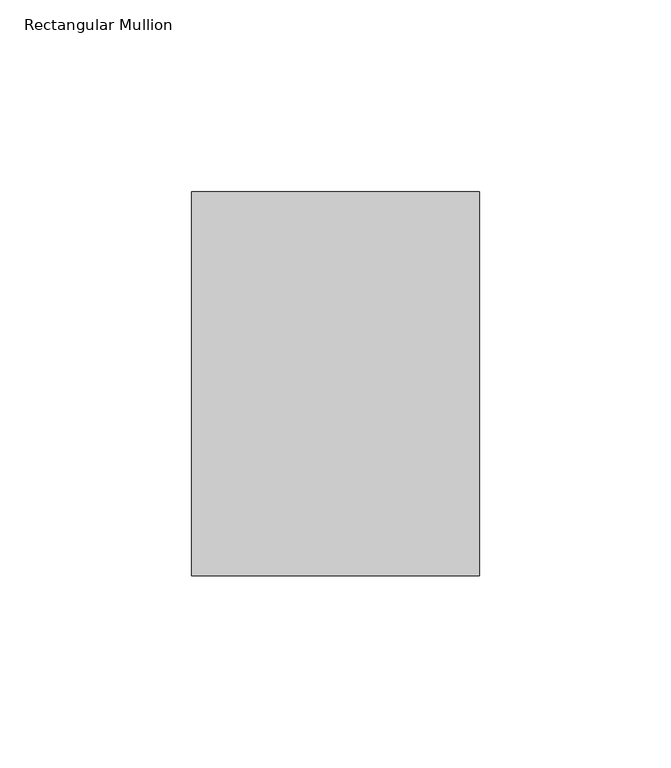
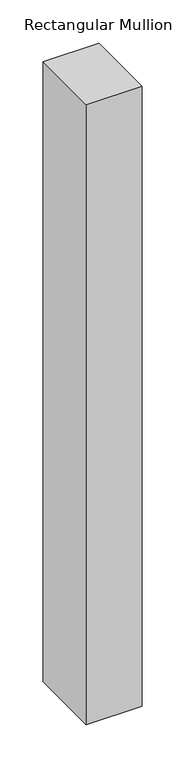
"""IFC4 building model written with IfcOpenShell, lengths in millimetres: member geometry, Rectangular Mullion : 알루미늄_Rectangular Cap_100 x 75."""

from ifc_helpers import new_model, si_unit, frame, origin, place, context, project, spatial, polyline, outline, extrude, source, transform, mapped, element, save


def rectangular_mullion_fe860069(model_context):
    return source(origin(), model_context, "Body", "SweptSolid", [
        extrude(outline(polyline([(0.0, 50.0), (0.0, -50.0), (-75.0, -50.0), (-75.0, 50.0), (0.0, 50.0)])), frame((0.0, 0.0, -877.5), z_axis=(0.0, 0.0, 1.0), x_axis=(1.0, 0.0, 0.0)), (0.0, 0.0, 1.0), 877.5),
    ])


if __name__ == "__main__":
    model = new_model("IFC4")
    model_context = context("Model", 3, world=origin())
    ifc_project = project(units=[si_unit("LENGTHUNIT", "METRE", prefix="MILLI")], contexts=[model_context])
    site = spatial("IfcSite", under=ifc_project)
    building = spatial("IfcBuilding", under=site)
    placement = place(None, origin())
    rectangular_mullion_shape = rectangular_mullion_fe860069(model_context)
    element("IfcMember", 1, ObjectType="Rectangular Mullion : 알루미늄_Rectangular Cap_100 x 75", at=placement, inside=building, context=model_context, shape_type="MappedRepresentation", body=[
        mapped(rectangular_mullion_shape, transform((0.0, 0.0, 0.0), x_axis=(1.0, 0.0, 0.0), y_axis=(0.0, 1.0, 0.0), z_axis=(0.0, 0.0, 1.0))),
    ])
    save(model, "model.ifc")

# Revit data of these elements
# Type "Rectangular Mullion : 알루미늄_Rectangular Cap_100 x 75"
#   built-in parameter 1007304 = 0.328084 (stored number, unit not read)
#   built-in parameter 1007301 = 0.123031 (stored number, unit not read)
#   built-in parameter 1007300 = 0.123031 (stored number, unit not read)
# Element 1 (IfcMember, "Rectangular Mullion : 알루미늄_Rectangular Cap_100 x 75")
#   Materials on its faces: "00_Metal_Stainless Steel"
# Materials
#   "00_Metal_Stainless Steel": class "Metal", colour RGB 148 148 148, transparency 0, Description = "Steel", Cost = 0
